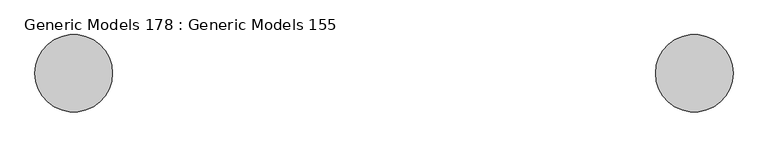
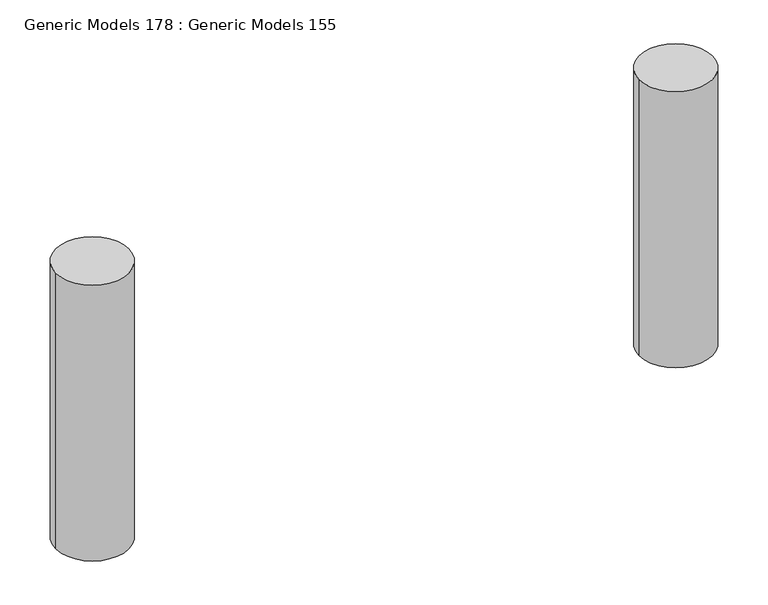
"""IFC4 building model written with IfcOpenShell, lengths in millimetres: proxy geometry, Generic Models 178 : Generic Models 155."""

from ifc_helpers import new_model, si_unit, point, frame, frame_2d, origin, place, context, project, spatial, circle_curve, trimmed, segment, composite_curve, outline, extrude, source, transform, mapped, element, save


def generic_models_178_generic_models_155_a54ccf4c(model_context):
    return source(origin(), model_context, "Body", "SweptSolid", [
        extrude(outline(composite_curve([segment(trimmed(circle_curve(frame_2d((56595.9625, 458.7875)), 152.4), [point((56443.5625, 458.7875))], [point((56748.3625, 458.7875))], False, "CARTESIAN"), True, "CONTINUOUS"), segment(trimmed(circle_curve(frame_2d((56595.9625, 458.7875)), 152.4), [point((56748.3625, 458.7875))], [point((56443.5625, 458.7875))], False, "CARTESIAN"), True, "CONTINUOUS")], self_intersect=False)), frame((0.0, 0.0, -1219.2), z_axis=(0.0, 0.0, 1.0), x_axis=(1.0, 0.0, 0.0)), (0.0, 0.0, 1.0), 1219.2),
        extrude(outline(composite_curve([segment(trimmed(circle_curve(frame_2d((54157.5625, 458.7875)), 152.4), [point((54005.1625, 458.7875))], [point((54309.9625, 458.7875))], False, "CARTESIAN"), True, "CONTINUOUS"), segment(trimmed(circle_curve(frame_2d((54157.5625, 458.7875)), 152.4), [point((54309.9625, 458.7875))], [point((54005.1625, 458.7875))], False, "CARTESIAN"), True, "CONTINUOUS")], self_intersect=False)), frame((0.0, 0.0, -1219.2), z_axis=(0.0, 0.0, 1.0), x_axis=(1.0, 0.0, 0.0)), (0.0, 0.0, 1.0), 1219.2),
    ])


if __name__ == "__main__":
    model = new_model("IFC4")
    model_context = context("Model", 3, world=origin())
    ifc_project = project(units=[si_unit("LENGTHUNIT", "METRE", prefix="MILLI")], contexts=[model_context])
    site = spatial("IfcSite", under=ifc_project)
    building = spatial("IfcBuilding", under=site)
    placement = place(None, origin())
    generic_models_178_generic_models_155_shape = generic_models_178_generic_models_155_a54ccf4c(model_context)
    element("IfcBuildingElementProxy", 1, Name="Generic Models 178 : Generic Models 155", ObjectType="Generic Models 178 : Generic Models 155", at=placement, inside=building, context=model_context, shape_type="MappedRepresentation", body=[
        mapped(generic_models_178_generic_models_155_shape, transform((0.0, 0.0, 0.0), x_axis=(1.0, 0.0, 0.0), y_axis=(0.0, 1.0, 0.0), z_axis=(0.0, 0.0, 1.0))),
    ])
    save(model, "model.ifc")

# Revit data of these elements
# Element 1 (IfcBuildingElementProxy, "Generic Models 178 : Generic Models 155")
#   Materials on its faces: "CONCRETE (3000 PSI CONCRETE)"
# Materials
#   "CONCRETE (3000 PSI CONCRETE)": class "Concrete", colour RGB 192 192 192, transparency 0, Description = "Cast-in-place concrete", Cost = 0
